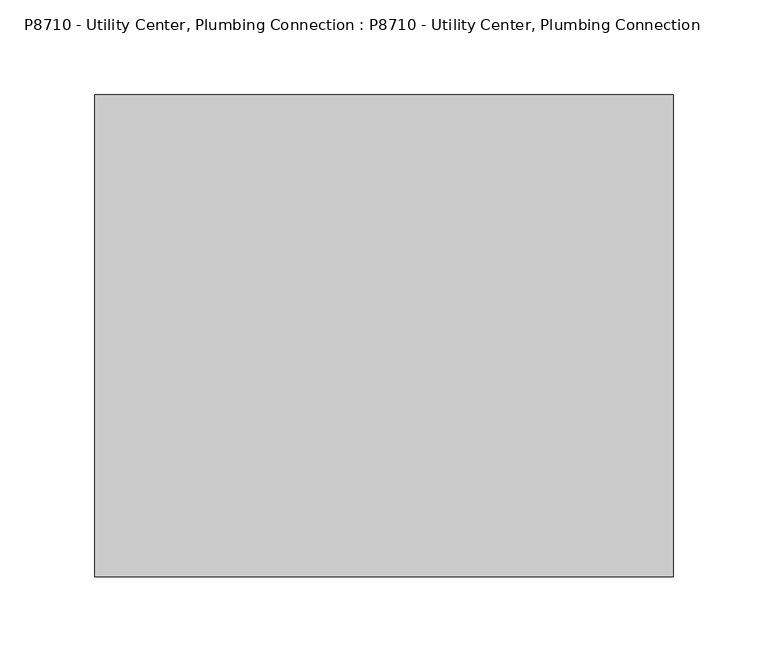
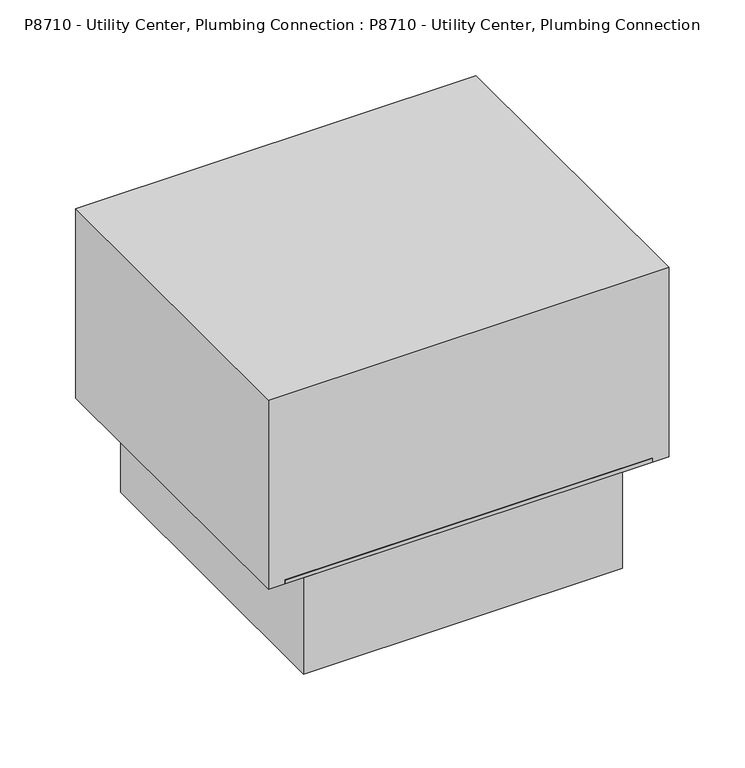
"""IFC4 building model written with IfcOpenShell, lengths in millimetres: proxy geometry, P8710 - Utility Center, Plumbing Connection : P8710 - Utility Center, Plumbing Connection."""

from ifc_helpers import new_model, si_unit, origin, origin_with_axes, place, context, project, spatial, polyline, outline, extrude, faceted_brep, source, transform, mapped, element, save


def p8710_utility_center_plumbing_connection_p8710_utility_0cc56990(model_context):
    return source(origin(), model_context, "Body", "SolidModel", [
        faceted_brep([(139.7, 127.0, 3.175), (-139.7, 127.0, 3.175), (-139.7, -127.0, 3.175), (139.7, -127.0, 3.175), (114.3, -101.6, 3.175), (-114.3, -101.6, 3.175), (-114.3, 101.9737484, 3.175), (114.3, 101.9737484, 3.175), (139.7, 127.0, 0.0), (139.7, -127.0, 0.0), (-139.7, -127.0, 0.0), (-139.7, 127.0, 0.0), (120.65, -120.65, 0.0), (120.65, 120.65, 0.0), (-122.0738096, 120.65, 0.0), (-122.0738096, -120.65, 0.0), (120.65, -120.65, -82.55), (120.65, 120.65, -82.55), (-122.0738096, 120.65, -82.55), (-122.0738096, -120.65, -82.55), (114.3, -101.6, -76.2), (-114.3, -101.6, -76.2), (-114.3, 101.9737484, -76.2), (114.3, 101.9737484, -76.2)], [[[0, 1, 2, 3], [4, 5, 6, 7]], [[8, 9, 10, 11], [12, 13, 14, 15]], [[1, 0, 8, 11]], [[2, 1, 11, 10]], [[3, 2, 10, 9]], [[0, 3, 9, 8]], [[12, 16, 17, 13]], [[14, 18, 19, 15]], [[16, 12, 15, 19]], [[17, 16, 19, 18]], [[13, 17, 18, 14]], [[4, 20, 21, 5]], [[6, 22, 23, 7]], [[5, 21, 22, 6]], [[21, 20, 23, 22]], [[20, 4, 7, 23]]]),
        extrude(outline(polyline([(152.4, 127.0), (152.4, -127.0), (-152.4, -127.0), (-152.4, 127.0), (152.4, 127.0)])), origin_with_axes(), (0.0, 0.0, 1.0), 152.4),
    ])


if __name__ == "__main__":
    model = new_model("IFC4")
    model_context = context("Model", 3, world=origin())
    ifc_project = project(units=[si_unit("LENGTHUNIT", "METRE", prefix="MILLI")], contexts=[model_context])
    site = spatial("IfcSite", under=ifc_project)
    building = spatial("IfcBuilding", under=site)
    placement = place(None, origin())
    p8710_utility_center_plumbing_connection_p8710_utility_shape = p8710_utility_center_plumbing_connection_p8710_utility_0cc56990(model_context)
    element("IfcBuildingElementProxy", 1, Name="P8710 - Utility Center, Plumbing Connection : P8710 - Utility Center, Plumbing Connection", ObjectType="P8710 - Utility Center, Plumbing Connection : P8710 - Utility Center, Plumbing Connection", at=placement, inside=building, context=model_context, shape_type="MappedRepresentation", body=[
        mapped(p8710_utility_center_plumbing_connection_p8710_utility_shape, transform((0.0, 0.0, 0.0), x_axis=(1.0, 0.0, 0.0), y_axis=(0.0, 1.0, 0.0), z_axis=(0.0, 0.0, 1.0))),
    ])
    save(model, "model.ifc")

# Revit data of these elements
# Project information
#   Room Abbreviation = "LDRP1"
#   Room Description 3-1 = "Labor & Delivery Room (LDRP1)"
#   Room Description 3-2 = "Storage Room, Equipment/Shelving (SRSE1)"
#   Room Description 3-3 = "Toilet/Shower (TLTS2)"
#   Sheets - Total = "9"
#   Project Issue Date = "Issue Date"
#   Project Status = "Project Status"
#   Client Name = "Owner"
#   Project Address = "Enter address here"
#   Project Name = "Project Name"
#   Project Number = "Project Number"
#   Publication Date = "30-Jan-15"
# Type "P8710 - Utility Center, Plumbing Connection : P8710 - Utility Center, Plumbing Connection"
#   Watts2 = "0"
#   Watts1 = "0"
#   Unit_Issue = "EA"
#   UTIL_6_Misc = "-"
#   UTIL_5_NonMedGas = "-"
#   UTIL_4_MiscGas = "-"
#   UTIL_3_MedGas = "-"
#   UTIL_2_Elec = "-"
#   UTIL_1_WaterDrain = "D"
#   Nomenclature = "Utility Center, Plumbing Connection"
#   NSN = "4100"
#   Location [instance default] = ""
#   JSN = "P8710"
#   Fund_Source_VA = "-"
#   Fund_Source_Navy = "-"
#   Fund_Source_Army = "-"
#   Fund_Source_AF = "-"
#   ELEC_Volts2 = "0"
#   ELEC_Volts1 = "0"
#   ELEC_Phase2 = "0"
#   ELEC_Phase1 = "0"
#   ELEC_HertzSwitch = "0"
#   ELEC_HertzDependent = "0"
#   ELEC_Hertz = "0"
#   ELEC_Amps2 = "0"
#   ELEC_Amps1 = "0"
#   DetailDescription = "Plumbing connection utility center, sometimes referred to as a ''GUY GRAY BOX''. This recessed utility center provides for hot and cold water connections and a drain connection at sink and other equipment locations. The utility center includes cutoff valves for the water connections, a plug seal for the drain and an outside cover to provide an aesthetic appearance when connections are no longer required.  This center may be installed in locations where no plumbing fixtures are included in a design as a future flexibility device, saving many dollars for later facility modifications to incorporate sinks as functions change."
#   CAT_VA = "A"
#   CAT_Navy = "A"
#   CAT_IHS = "-"
#   CAT_Army = "A"
#   CAT_AF = "A"
#   BTUperhour = "0"
#   Weight_IP = 10
#   Default Elevation = 4' - 6"
#   DIM_Width_IP = 1' - 0"
#   DIM_Height_IP = 0' - 10"
#   DIM_Depth_IP = 0' - 6"
#   Assembly Code = ""
# Element 1 (IfcBuildingElementProxy, "P8710 - Utility Center, Plumbing Connection : P8710 - Utility Center, Plumbing Connection")
#   Materials on its faces: "Finish", "EquipSpace"
# Materials
#   "Finish": class "Plastic", colour RGB 245 239 218, transparency 0
#   "EquipSpace": class "Unassigned", colour RGB 221 217 195, transparency 0.5
